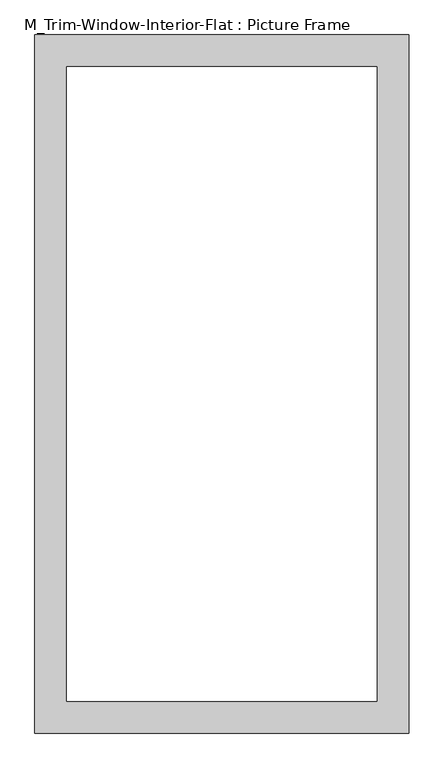
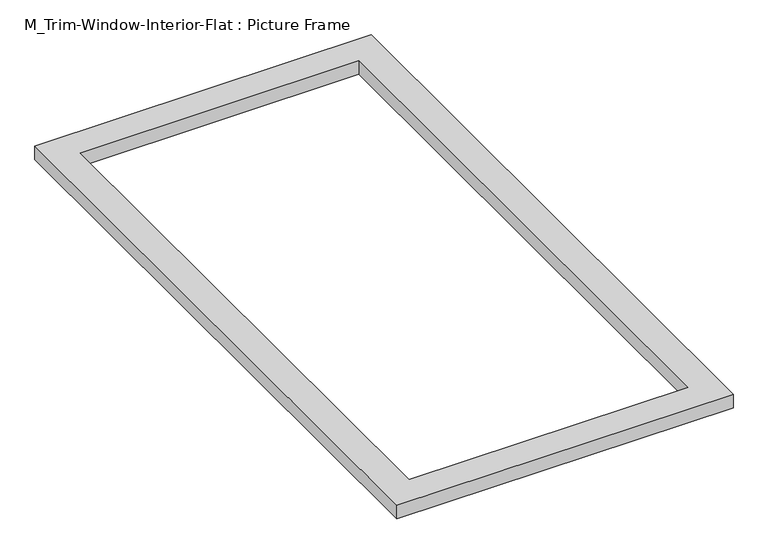
"""IFC4 building model written with IfcOpenShell, lengths in millimetres: proxy geometry, M_Trim-Window-Interior-Flat : Picture Frame."""

from ifc_helpers import new_model, si_unit, origin, origin_with_axes, place, context, project, spatial, polyline, outline, extrude, source, transform, mapped, element, save


def m_trim_window_interior_flat_picture_frame_b7ef0147(model_context):
    return source(origin(), model_context, "Body", "SweptSolid", [
        extrude(outline(polyline([(352.1, -47.3), (-352.1, -47.3), (-352.1, 1266.5), (352.1, 1266.5), (352.1, -47.3)]), holes=[polyline([(292.1, 12.7), (292.1, 1206.5), (-292.1, 1206.5), (-292.1, 12.7), (292.1, 12.7)])]), origin_with_axes(), (0.0, 0.0, 1.0), 30.0),
    ])


if __name__ == "__main__":
    model = new_model("IFC4")
    model_context = context("Model", 3, world=origin())
    ifc_project = project(units=[si_unit("LENGTHUNIT", "METRE", prefix="MILLI")], contexts=[model_context])
    site = spatial("IfcSite", under=ifc_project)
    building = spatial("IfcBuilding", under=site)
    placement = place(None, origin())
    m_trim_window_interior_flat_picture_frame_shape = m_trim_window_interior_flat_picture_frame_b7ef0147(model_context)
    element("IfcBuildingElementProxy", 1, Name="M_Trim-Window-Interior-Flat : Picture Frame", ObjectType="M_Trim-Window-Interior-Flat : Picture Frame", at=placement, inside=building, context=model_context, shape_type="MappedRepresentation", body=[
        mapped(m_trim_window_interior_flat_picture_frame_shape, transform((0.0, 0.0, 0.0), x_axis=(1.0, 0.0, 0.0), y_axis=(0.0, 1.0, 0.0), z_axis=(0.0, 0.0, 1.0))),
    ])
    save(model, "model.ifc")

# Revit data of these elements
# Type "M_Trim-Window-Interior-Flat : Picture Frame"
#   Trim Thickness_Picture Frame = 0' - 1.1811"
#   Trim Width = 0' - 2.3622"
#   Trim Thickness_with Sill = 0' - 0.7874"
#   Sill Thickness = 0' - 1.1811"
#   Opening Width [instance default] = 1' - 11.62205"
#   Opening Height [instance default] = 2' - 11.43307"
#   Default Elevation = 3' - 11.24409"
#   Sill = no
#   Picture Frame = yes
#   Trim Material [instance default] = none
# Element 1 (IfcBuildingElementProxy, "M_Trim-Window-Interior-Flat : Picture Frame")
#   Opening Width = 2' - 0"
#   Opening Height = 4' - 0"
#   Trim Material = Wood - Stained
#   Materials on its faces: "Wood - Stained"
# Materials
#   "Wood - Stained": class "Wood", colour RGB 224 178 126, transparency 0, Cost = 0
